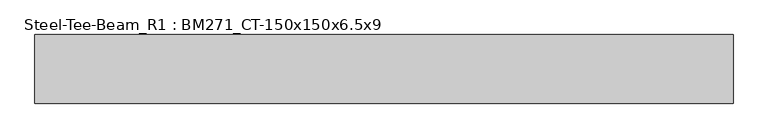
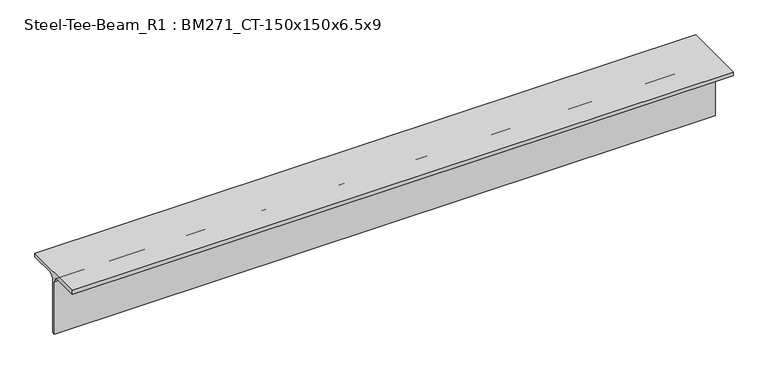
"""IFC4 building model written with IfcOpenShell, lengths in millimetres: member geometry, Steel-Tee-Beam_R1 : BM271_CT-150x150x6.5x9."""

from ifc_helpers import new_model, si_unit, point, frame, frame_2d, origin, place, context, project, spatial, polyline, circle_curve, trimmed, segment, composite_curve, outline, extrude, source, transform, mapped, element, save


def steel_tee_beam_r1_bm271_ct_150x150x6_5x9_f5588b02(model_context):
    return source(origin(), model_context, "Body", "SweptSolid", [
        extrude(outline(composite_curve([segment(polyline([(-75.0, 75.0), (75.0, 75.0), (75.0, 66.0), (16.25, 66.0)]), True, "CONTINUOUS"), segment(trimmed(circle_curve(frame_2d((16.25, 53.0)), 13.0), [point((16.25, 66.0))], [point((3.25, 53.0))], True, "CARTESIAN"), True, "CONTINUOUS"), segment(polyline([(3.25, 53.0), (3.25, -75.0), (-3.25, -75.0), (-3.25, 53.0)]), True, "CONTINUOUS"), segment(trimmed(circle_curve(frame_2d((-16.25, 53.0)), 13.0), [point((-3.25, 53.0))], [point((-16.25, 66.0))], True, "CARTESIAN"), True, "CONTINUOUS"), segment(polyline([(-16.25, 66.0), (-75.0, 66.0), (-75.0, 75.0)]), True, "CONTINUOUS")], self_intersect=False)), frame((-719.0402776, 0.0, 0.0), z_axis=(1.0, 0.0, 0.0), x_axis=(0.0, 1.0, 0.0)), (0.0, 0.0, 1.0), 1526.1440409),
    ])


if __name__ == "__main__":
    model = new_model("IFC4")
    model_context = context("Model", 3, world=origin())
    ifc_project = project(units=[si_unit("LENGTHUNIT", "METRE", prefix="MILLI")], contexts=[model_context])
    site = spatial("IfcSite", under=ifc_project)
    building = spatial("IfcBuilding", under=site)
    placement = place(None, origin())
    steel_tee_beam_r1_bm271_ct_150x150x6_5x9_shape = steel_tee_beam_r1_bm271_ct_150x150x6_5x9_f5588b02(model_context)
    element("IfcMember", 1, ObjectType="Steel-Tee-Beam_R1 : BM271_CT-150x150x6.5x9", at=placement, inside=building, context=model_context, shape_type="MappedRepresentation", body=[
        mapped(steel_tee_beam_r1_bm271_ct_150x150x6_5x9_shape, transform((0.0, 0.0, 0.0), x_axis=(1.0, 0.0, 0.0), y_axis=(0.0, 1.0, 0.0), z_axis=(0.0, 0.0, 1.0))),
    ])
    save(model, "model.ifc")

# Revit data of these elements
# Type "Steel-Tee-Beam_R1 : BM271_CT-150x150x6.5x9"
#   Keynote = "CT-150x150x6.5x9"
#   Surface Area = 0.588841 m²/m
#   Section Area = 23.3904 cm²
#   Mass per Unit Length = 18.3614 kg/m
#   Length [instance default] = 1.5240 m
#   bf = 0.1500 m
#   d = 0.1500 m
#   k = 0.0220 m
#   r = 0.0130 m
#   tf = 0.0090 m
#   tw = 0.0065 m
#   hec_material4 [instance default] = none
#   hec_material3 [instance default] = none
#   hec_material2 [instance default] = none
#   hec_material1 [instance default] = none
#   Structural Material [instance default] = Steel, 45-345
#   Assembly Code = ""
# Element 1 (IfcMember, "Steel-Tee-Beam_R1 : BM271_CT-150x150x6.5x9")
#   Structural Material = none
# Materials
#   "Steel, 45-345": class "Metal", colour RGB 189 187 185, transparency 0, Description = "Steel 345 MPa", Cost = 0
